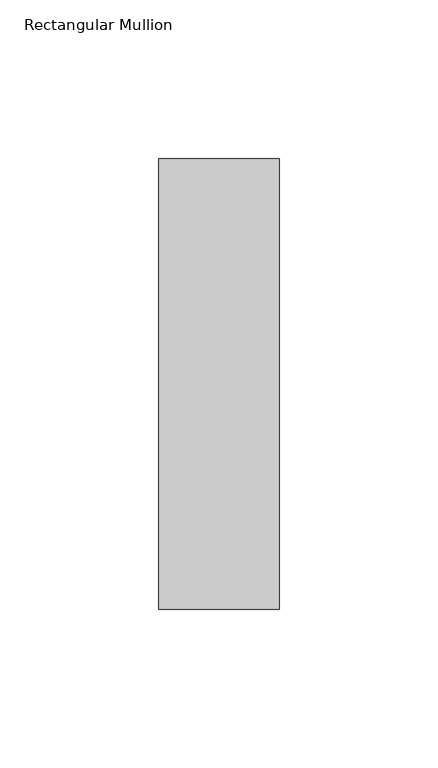
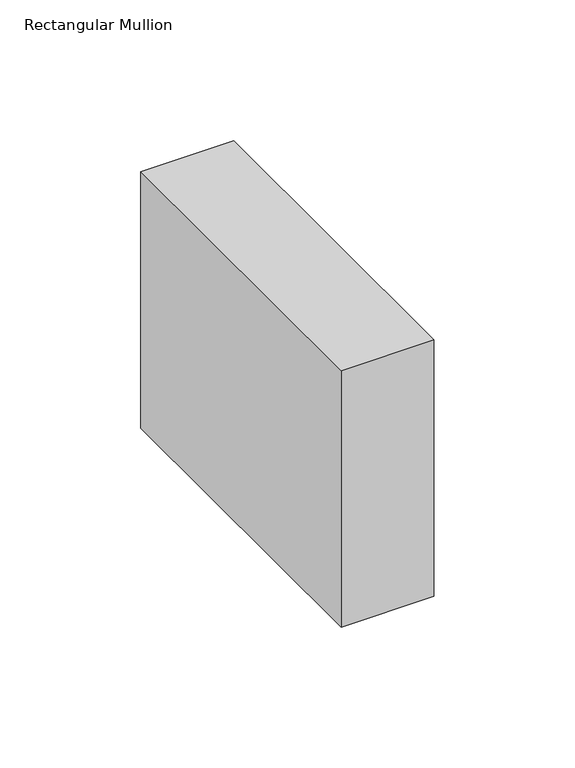
"""IFC4 building model written with IfcOpenShell, lengths in millimetres: member geometry, Rectangular Mullion : NLRS_21_CWM_hsb-regel 38x142_gen_rsf."""

from ifc_helpers import new_model, si_unit, frame, origin, place, context, project, spatial, polyline, outline, extrude, source, transform, mapped, element, save


def rectangular_mullion_8b5cfd33(model_context):
    return source(origin(), model_context, "Body", "SweptSolid", [
        extrude(outline(polyline([(0.0, -71.0), (-38.0, -71.0), (-38.0, 71.0), (0.0, 71.0), (0.0, -71.0)])), frame((0.0, 0.0, -111.0), z_axis=(0.0, 0.0, 1.0), x_axis=(1.0, 0.0, 0.0)), (0.0, 0.0, 1.0), 111.0),
    ])


if __name__ == "__main__":
    model = new_model("IFC4")
    model_context = context("Model", 3, world=origin())
    ifc_project = project(units=[si_unit("LENGTHUNIT", "METRE", prefix="MILLI")], contexts=[model_context])
    site = spatial("IfcSite", under=ifc_project)
    building = spatial("IfcBuilding", under=site)
    placement = place(None, origin())
    rectangular_mullion_shape = rectangular_mullion_8b5cfd33(model_context)
    element("IfcMember", 1, ObjectType="Rectangular Mullion : NLRS_21_CWM_hsb-regel 38x142_gen_rsf", at=placement, inside=building, context=model_context, shape_type="MappedRepresentation", body=[
        mapped(rectangular_mullion_shape, transform((0.0, 0.0, 0.0), x_axis=(1.0, 0.0, 0.0), y_axis=(0.0, 1.0, 0.0), z_axis=(0.0, 0.0, 1.0))),
    ])
    save(model, "model.ifc")

# Revit data of these elements
# Type "Rectangular Mullion : NLRS_21_CWM_hsb-regel 38x142_gen_rsf"
#   Export Type to IFC As = "IfcWall"
#   Type IfcGUID = "07M7mRoiH1CR8m_RSKIwpF"
#   Assembly Code = "21.10"
#   built-in parameter 1007322 = 0.465879 (stored number, unit not read)
#   built-in parameter 1007321 = 0.062336 (stored number, unit not read)
#   built-in parameter 1007320 = 0.062336 (stored number, unit not read)
# Element 1 (IfcMember, "Rectangular Mullion : NLRS_21_CWM_hsb-regel 38x142_gen_rsf")
#   Materials on its faces: "NLRS_i2_hout naaldhout vuren_gen_rsf"
# Materials
#   "NLRS_i2_hout naaldhout vuren_gen_rsf": class "I - Hout", colour RGB 234 199 147, transparency 0, Keynote = "i2", Manufacturer = "Revit Standards Foundation", URL = "www.revitstandards.org", Description = "hout vuren", Cost = 0
